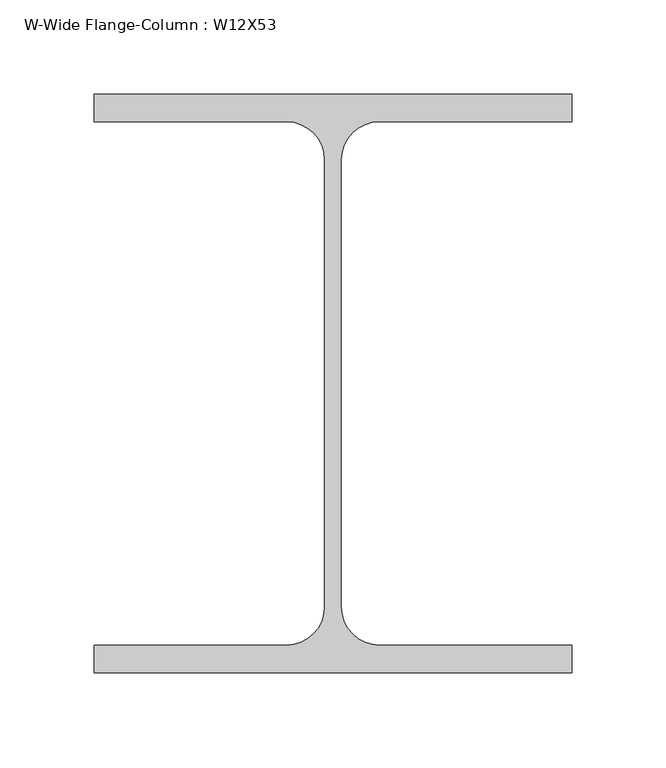
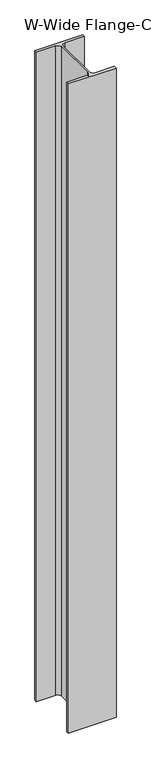
"""IFC4 building model written with IfcOpenShell, lengths in millimetres: column geometry, W-Wide Flange-Column : W12X53."""

from ifc_helpers import new_model, si_unit, point, frame, frame_2d, origin, place, context, project, spatial, polyline, circle_curve, trimmed, segment, composite_curve, outline, extrude, source, transform, mapped, element, save


def w_wide_flange_column_w12x53_6c22db8c(model_context):
    return source(origin(), model_context, "Body", "SweptSolid", [
        extrude(outline(composite_curve([segment(polyline([(127.0, 153.67), (127.0, 139.065), (24.7015, 139.065)]), True, "CONTINUOUS"), segment(trimmed(circle_curve(frame_2d((24.7015, 118.745)), 20.32), [point((24.7015, 139.065))], [point((4.3815, 118.745))], True, "CARTESIAN"), True, "CONTINUOUS"), segment(polyline([(4.3815, 118.745), (4.3815, -118.745)]), True, "CONTINUOUS"), segment(trimmed(circle_curve(frame_2d((24.7015, -118.745)), 20.32), [point((4.3815, -118.745))], [point((24.7015, -139.065))], True, "CARTESIAN"), True, "CONTINUOUS"), segment(polyline([(24.7015, -139.065), (127.0, -139.065), (127.0, -153.67), (-127.0, -153.67), (-127.0, -139.065), (-24.7015, -139.065)]), True, "CONTINUOUS"), segment(trimmed(circle_curve(frame_2d((-24.7015, -118.745)), 20.32), [point((-24.7015, -139.065))], [point((-4.3815, -118.745))], True, "CARTESIAN"), True, "CONTINUOUS"), segment(polyline([(-4.3815, -118.745), (-4.3815, 118.745)]), True, "CONTINUOUS"), segment(trimmed(circle_curve(frame_2d((-24.7015, 118.745)), 20.32), [point((-4.3815, 118.745))], [point((-24.7015, 139.065))], True, "CARTESIAN"), True, "CONTINUOUS"), segment(polyline([(-24.7015, 139.065), (-127.0, 139.065), (-127.0, 153.67), (127.0, 153.67)]), True, "CONTINUOUS")], self_intersect=False)), frame((0.0, 0.0, 8756.65), z_axis=(0.0, 0.0, 1.0), x_axis=(1.0, 0.0, 0.0)), (0.0, 0.0, 1.0), 3651.25),
    ])


if __name__ == "__main__":
    model = new_model("IFC4")
    model_context = context("Model", 3, world=origin())
    ifc_project = project(units=[si_unit("LENGTHUNIT", "METRE", prefix="MILLI")], contexts=[model_context])
    site = spatial("IfcSite", under=ifc_project)
    building = spatial("IfcBuilding", under=site)
    placement = place(None, origin())
    w_wide_flange_column_w12x53_shape = w_wide_flange_column_w12x53_6c22db8c(model_context)
    element("IfcColumn", 1, ObjectType="W-Wide Flange-Column : W12X53", at=placement, inside=building, context=model_context, shape_type="MappedRepresentation", body=[
        mapped(w_wide_flange_column_w12x53_shape, transform((0.0, 0.0, 0.0), x_axis=(1.0, 0.0, 0.0), y_axis=(0.0, 1.0, 0.0), z_axis=(0.0, 0.0, 1.0))),
    ])
    save(model, "model.ifc")

# Revit data of these elements
# Type "W-Wide Flange-Column : W12X53"
#   Assembly Code = "B10"
#   W = 53
#   bf = 0' - 10"
#   d = 1' - 0.1"
#   k = 0' - 1 3/8"
#   kr = 0' - 0.8"
#   tf = 0' - 0.575"
#   tw = 0' - 0.345"
#   A = 0.108333 SF
#   Structural Material [instance default] = Steel ASTM A992
# Element 1 (IfcColumn, "W-Wide Flange-Column : W12X53")
#   Materials on its faces: "Steel ASTM A992"
# Materials
#   "Steel ASTM A992": class "Metal", colour RGB 199 199 199, transparency 0, Description = "Structural steel 50ksi", Cost = 0
